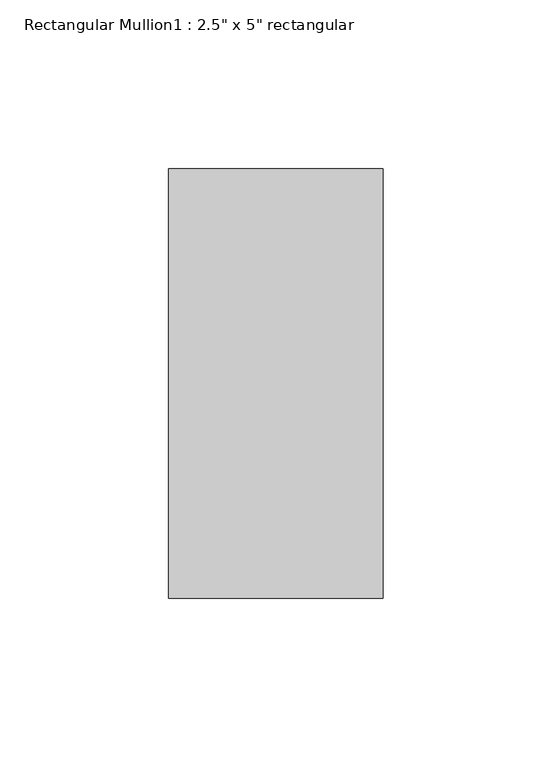
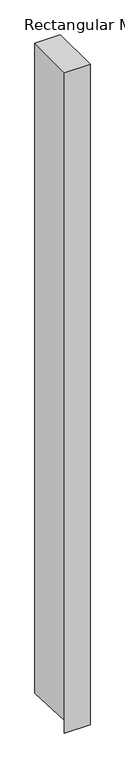
"""IFC4 building model written with IfcOpenShell, lengths in millimetres: member geometry."""

from ifc_helpers import new_model, si_unit, frame, origin, place, context, project, spatial, polyline, outline, extrude, source, transform, mapped, element, save


def member_a8d07153(model_context):
    return source(origin(), model_context, "Body", "SweptSolid", [
        extrude(outline(polyline([(-63.5, 0.0), (63.5, 0.0), (63.5, -1705.0231573), (-62.1974623, -1700.0584389), (-63.5, -1733.0362781), (-63.5, 0.0)])), frame((-63.5, 0.0, 0.0), z_axis=(1.0, 0.0, 0.0), x_axis=(0.0, 1.0, 0.0)), (0.0, 0.0, 1.0), 63.5),
    ])


if __name__ == "__main__":
    model = new_model("IFC4")
    model_context = context("Model", 3, world=origin())
    ifc_project = project(units=[si_unit("LENGTHUNIT", "METRE", prefix="MILLI")], contexts=[model_context])
    site = spatial("IfcSite", under=ifc_project)
    building = spatial("IfcBuilding", under=site)
    placement = place(None, origin())
    member_shape = member_a8d07153(model_context)
    element("IfcMember", 1, ObjectType="Rectangular Mullion1 : 2.5\" x 5\" rectangular", at=placement, inside=building, context=model_context, shape_type="MappedRepresentation", body=[
        mapped(member_shape, transform((0.0, 0.0, 0.0), x_axis=(1.0, 0.0, 0.0), y_axis=(0.0, 1.0, 0.0), z_axis=(0.0, 0.0, 1.0))),
    ])
    save(model, "model.ifc")

# Revit data of these elements
# Type "Rectangular Mullion1 : 2.5\" x 5\" rectangular"
#   built-in parameter 1007304 = 0.416667 (stored number, unit not read)
#   built-in parameter 1007301 = 0.104167 (stored number, unit not read)
#   built-in parameter 1007300 = 0.104167 (stored number, unit not read)
# Element 1 (IfcMember, "Rectangular Mullion1 : 2.5\" x 5\" rectangular")
#   Materials on its faces: "support-frame"
# Materials
#   "support-frame": class "Unassigned", colour RGB 233 233 233, transparency 0, Cost = 0
